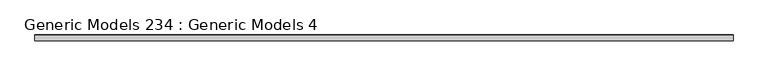
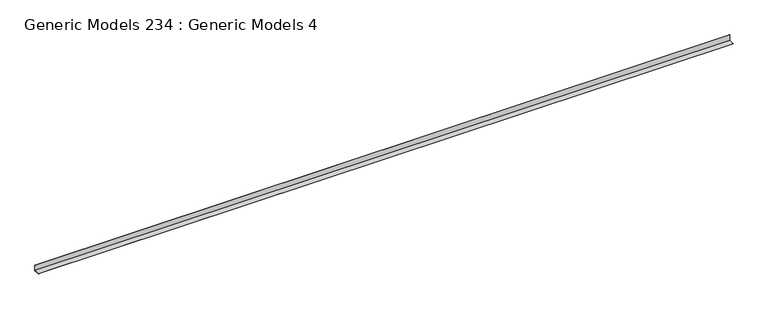
"""IFC4 building model written with IfcOpenShell, lengths in millimetres: proxy geometry, Generic Models 234 : Generic Models 4."""

import ifcopenshell
import ifcopenshell.guid

model = None  # the IFC model being written
_history = None  # IfcOwnerHistory: only IFC2X3 demands one
_inside = {}  # id of a spatial element -> (the spatial element, [elements in it])
_under = {}  # id of a project, library or spatial element -> (it, [spatial elements below it])
_declared = {}  # id of a project -> (the project, [libraries it declares])
_typed = {}  # id of a type object -> (the type object, [elements of that type])
_made_of = {}  # id of a material, layer set ... -> (it, [elements and type objects made of it])


def new_model(schema):
    """Start an empty IFC model of exactly this schema.

    Asked for "IFC4X3", IfcOpenShell would pick the latest addendum, in which some entities
    have other attributes; the version numbers below select the first issue.
    IFC2X3 requires an IfcOwnerHistory on every rooted entity: one is made here for all.
    """
    global model, _history
    if schema == "IFC4X3":
        model = ifcopenshell.file(schema_version=(4, 3, 0, 0))
    else:
        model = ifcopenshell.file(schema=schema)
    _inside.clear()
    _under.clear()
    _declared.clear()
    _typed.clear()
    _made_of.clear()
    _history = None
    if model.schema == "IFC2X3":
        org = make("IfcOrganization", Name="unknown")
        user = make(
            "IfcPersonAndOrganization",
            ThePerson=make("IfcPerson", FamilyName="unknown"),
            TheOrganization=org,
        )
        app = make(
            "IfcApplication",
            ApplicationDeveloper=org,
            Version="unknown",
            ApplicationFullName="unknown",
            ApplicationIdentifier="unknown",
        )
        _history = make(
            "IfcOwnerHistory",
            OwningUser=user,
            OwningApplication=app,
            ChangeAction="ADDED",
            CreationDate=0,
        )
    return model


def make(cls, **values):
    """One entity of the class cls with the attributes given. An attribute that is None is left unset."""
    return model.create_entity(
        cls, **{name: value for name, value in values.items() if value is not None}
    )


def rooted(cls, **values):
    """An entity with a GlobalId (a new one), such as an element, a storey or a relation."""
    return make(cls, GlobalId=ifcopenshell.guid.new(), OwnerHistory=_history, **values)


def si_unit(unit_type, name, prefix=None):
    """IfcSIUnit, for example si_unit("LENGTHUNIT", "METRE", prefix="MILLI")."""
    return make("IfcSIUnit", UnitType=unit_type, Prefix=prefix, Name=name)


def assignment(units):
    """IfcUnitAssignment: the units of a project."""
    return None if units is None else make("IfcUnitAssignment", Units=units)


def point(xyz):
    """IfcCartesianPoint."""
    return None if xyz is None else make("IfcCartesianPoint", Coordinates=xyz)


def direction(xyz):
    """IfcDirection."""
    return None if xyz is None else make("IfcDirection", DirectionRatios=xyz)


def frame(location, z_axis=None, x_axis=None):
    """IfcAxis2Placement3D, a coordinate frame: its origin and axes. An axis left out is left unset."""
    return make(
        "IfcAxis2Placement3D",
        Location=point(location),
        Axis=direction(z_axis),
        RefDirection=direction(x_axis),
    )


def origin():
    """The frame at (0, 0, 0) with its axes left unset."""
    return frame((0.0, 0.0, 0.0))


def place(relative_to, where):
    """IfcLocalPlacement: puts the frame where relative to a parent placement (None: the world)."""
    return make(
        "IfcLocalPlacement", PlacementRelTo=relative_to, RelativePlacement=where
    )


def context(
    kind, dimensions, precision=None, world=None, true_north=None, identifier=None
):
    """IfcGeometricRepresentationContext, for example the 3D "Model" context."""
    return make(
        "IfcGeometricRepresentationContext",
        ContextIdentifier=identifier,
        ContextType=kind,
        CoordinateSpaceDimension=dimensions,
        Precision=precision,
        WorldCoordinateSystem=world,
        TrueNorth=true_north,
    )


def project(units=None, contexts=None):
    """IfcProject with its units and contexts."""
    return rooted(
        "IfcProject",
        Name="project",
        RepresentationContexts=contexts,
        UnitsInContext=assignment(units),
    )


def spatial(cls, under=None, at=None, **own):
    """A site, building, storey or space (cls), placed at a placement, below another one or the project."""
    s = rooted(cls, ObjectPlacement=at, **own)
    if under is not None:
        _under.setdefault(under.id(), (under, []))[1].append(s)
    return s


def polyline(points):
    """IfcPolyline through the points."""
    return make("IfcPolyline", Points=[point(p) for p in points])


def outline(outer, holes=None, kind="AREA"):
    """IfcArbitraryClosedProfileDef: a profile drawn as a closed curve; with holes, ...WithVoids."""
    if holes is None:
        return make("IfcArbitraryClosedProfileDef", ProfileType=kind, OuterCurve=outer)
    return make(
        "IfcArbitraryProfileDefWithVoids",
        ProfileType=kind,
        OuterCurve=outer,
        InnerCurves=holes,
    )


def extrude(swept, where, along, depth):
    """IfcExtrudedAreaSolid: the profile swept, set in the frame where, extruded along a direction by depth."""
    return make(
        "IfcExtrudedAreaSolid",
        SweptArea=swept,
        Position=where,
        ExtrudedDirection=direction(along),
        Depth=depth,
    )


def shape(context_of_items, identifier, shape_type, items):
    """IfcShapeRepresentation: the items that make up one representation, for example the "Body"."""
    return make(
        "IfcShapeRepresentation",
        ContextOfItems=context_of_items,
        RepresentationIdentifier=identifier,
        RepresentationType=shape_type,
        Items=items,
    )


def source(mapping_origin, context_of_items, identifier, shape_type, items):
    """IfcRepresentationMap: a shape defined once, which mapped items show again and again."""
    return make(
        "IfcRepresentationMap",
        MappingOrigin=mapping_origin,
        MappedRepresentation=shape(context_of_items, identifier, shape_type, items),
    )


def transform(
    local_origin,
    x_axis=None,
    y_axis=None,
    z_axis=None,
    scale=None,
    scale2=None,
    scale3=None,
    uniform=True,
):
    """IfcCartesianTransformationOperator3D, or its non-uniform kind. x_axis, y_axis, z_axis: its Axis1, 2, 3."""
    if uniform:
        return make(
            "IfcCartesianTransformationOperator3D",
            Axis1=direction(x_axis),
            Axis2=direction(y_axis),
            LocalOrigin=point(local_origin),
            Scale=scale,
            Axis3=direction(z_axis),
        )
    return make(
        "IfcCartesianTransformationOperator3DnonUniform",
        Axis1=direction(x_axis),
        Axis2=direction(y_axis),
        LocalOrigin=point(local_origin),
        Scale=scale,
        Axis3=direction(z_axis),
        Scale2=scale2,
        Scale3=scale3,
    )


def mapped(mapping_source, mapping_target):
    """IfcMappedItem: shows the shape of a source again, moved by a transform."""
    return make(
        "IfcMappedItem", MappingSource=mapping_source, MappingTarget=mapping_target
    )


def made_of(thing, what):
    """Note that an element or type object is made of a material, layer set ...; save() writes the relation."""
    if what is not None:
        _made_of.setdefault(what.id(), (what, []))[1].append(thing)
    return thing


def element(
    cls,
    number,
    at=None,
    inside=None,
    cuts=None,
    type_object=None,
    material=None,
    context=None,
    identifier="Body",
    shape_type=None,
    held_by="IfcProductDefinitionShape",
    body=None,
    shapes=None,
    **own,
):
    """One element of the class cls, such as IfcWall. Its Tag is "e" and its number.

    at: its placement. inside: the storey or other place that contains it. cuts: it is an
    opening in that element (IfcRelVoidsElement). A single representation is given by context,
    identifier, shape_type and body (its items); several are given by shapes. held_by: the class
    of the entity that holds the representations. save() writes the other relations.
    """
    e = rooted(cls, Tag="e%d" % number, ObjectPlacement=at, **own)
    if body is not None:
        shapes = [shape(context, identifier, shape_type, body)]
    if shapes is not None:
        e.Representation = make(held_by, Representations=shapes)
    if inside is not None:
        _inside.setdefault(inside.id(), (inside, []))[1].append(e)
    if cuts is not None:
        rooted(
            "IfcRelVoidsElement", RelatingBuildingElement=cuts, RelatedOpeningElement=e
        )
    if type_object is not None:
        _typed.setdefault(type_object.id(), (type_object, []))[1].append(e)
    return made_of(e, material)


def aggregate(whole, parts):
    """IfcRelAggregates: a whole, such as a stair, and the parts it consists of."""
    return rooted("IfcRelAggregates", RelatingObject=whole, RelatedObjects=parts)


def save(model, path):
    """Write the relations noted so far, then the file.

    IfcRelAggregates (storeys below a building ...), IfcRelContainedInSpatialStructure (elements
    in a storey), IfcRelDefinesByType, IfcRelAssociatesMaterial and IfcRelDeclares: one each for
    every whole, place, type object, material and project.
    """
    for whole, parts in _under.values():
        aggregate(whole, parts)
    for where, things in _inside.values():
        rooted(
            "IfcRelContainedInSpatialStructure",
            RelatedElements=things,
            RelatingStructure=where,
        )
    for kind, things in _typed.values():
        rooted("IfcRelDefinesByType", RelatedObjects=things, RelatingType=kind)
    for what, things in _made_of.values():
        rooted("IfcRelAssociatesMaterial", RelatedObjects=things, RelatingMaterial=what)
    for by, libraries in _declared.values():
        rooted("IfcRelDeclares", RelatingContext=by, RelatedDefinitions=libraries)
    model.write(path)


def generic_models_234_generic_models_4_41341a2f(model_context):
    return source(origin(), model_context, "Body", "SweptSolid", [
        extrude(outline(polyline([(11784.9929664, 126903.8965937), (11784.9929664, 127058.729047), (11785.7867164, 127058.729047), (11785.7867164, 126903.1028437), (11632.6093306, 126903.1028437), (11632.6093306, 126903.8965937), (11784.9929664, 126903.8965937)])), frame((-10234.5171316, 0.0, 0.0), z_axis=(1.0, 0.0, 0.0), x_axis=(0.0, 1.0, 0.0)), (0.0, 0.0, 1.0), 18643.6),
    ])


if __name__ == "__main__":
    model = new_model("IFC4")
    model_context = context("Model", 3, world=origin())
    ifc_project = project(units=[si_unit("LENGTHUNIT", "METRE", prefix="MILLI")], contexts=[model_context])
    site = spatial("IfcSite", under=ifc_project)
    building = spatial("IfcBuilding", under=site)
    placement = place(None, origin())
    generic_models_234_generic_models_4_shape = generic_models_234_generic_models_4_41341a2f(model_context)
    element("IfcBuildingElementProxy", 1, Name="Generic Models 234 : Generic Models 4", ObjectType="Generic Models 234 : Generic Models 4", at=placement, inside=building, context=model_context, shape_type="MappedRepresentation", body=[
        mapped(generic_models_234_generic_models_4_shape, transform((0.0, 0.0, 0.0), x_axis=(1.0, 0.0, 0.0), y_axis=(0.0, 1.0, 0.0), z_axis=(0.0, 0.0, 1.0))),
    ])
    save(model, "model.ifc")

# Revit data of these elements
# Element 1 (IfcBuildingElementProxy, "Generic Models 234 : Generic Models 4")
#   Materials on its faces: "_16 GA. COPPER \"L\" FLASHING - (6\" HORZ. LEG - 4\" VERT. LEG)"
# Materials
#   "_16 GA. COPPER \"L\" FLASHING - (6\" HORZ. LEG - 4\" VERT. LEG)": class "Generic", colour RGB 156 184 169, transparency 0, Cost = 0
